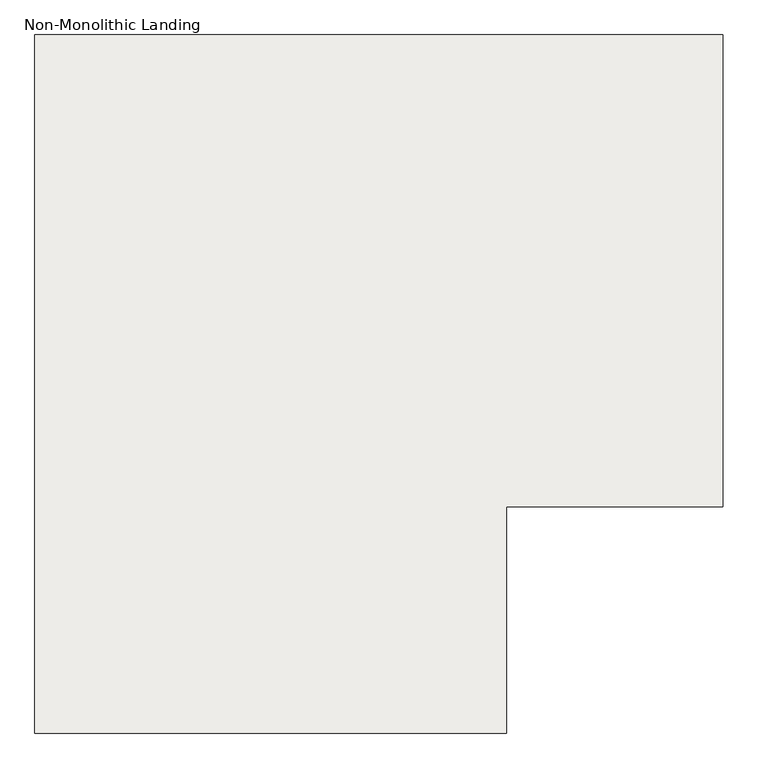
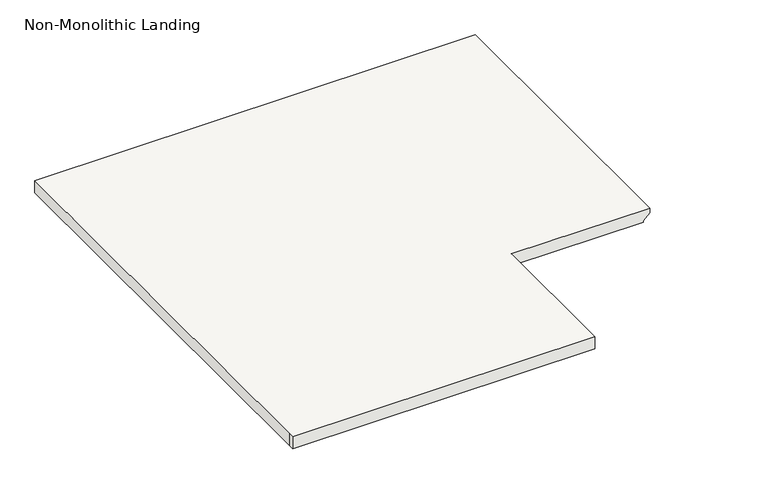
"""IFC4 building model written with IfcOpenShell, lengths in millimetres: slab geometry, Non-Monolithic Landing."""

import ifcopenshell
import ifcopenshell.guid

model = None  # the IFC model being written
_history = None  # IfcOwnerHistory: only IFC2X3 demands one
_inside = {}  # id of a spatial element -> (the spatial element, [elements in it])
_under = {}  # id of a project, library or spatial element -> (it, [spatial elements below it])
_declared = {}  # id of a project -> (the project, [libraries it declares])
_typed = {}  # id of a type object -> (the type object, [elements of that type])
_made_of = {}  # id of a material, layer set ... -> (it, [elements and type objects made of it])


def new_model(schema):
    """Start an empty IFC model of exactly this schema.

    Asked for "IFC4X3", IfcOpenShell would pick the latest addendum, in which some entities
    have other attributes; the version numbers below select the first issue.
    IFC2X3 requires an IfcOwnerHistory on every rooted entity: one is made here for all.
    """
    global model, _history
    if schema == "IFC4X3":
        model = ifcopenshell.file(schema_version=(4, 3, 0, 0))
    else:
        model = ifcopenshell.file(schema=schema)
    _inside.clear()
    _under.clear()
    _declared.clear()
    _typed.clear()
    _made_of.clear()
    _history = None
    if model.schema == "IFC2X3":
        org = make("IfcOrganization", Name="unknown")
        user = make(
            "IfcPersonAndOrganization",
            ThePerson=make("IfcPerson", FamilyName="unknown"),
            TheOrganization=org,
        )
        app = make(
            "IfcApplication",
            ApplicationDeveloper=org,
            Version="unknown",
            ApplicationFullName="unknown",
            ApplicationIdentifier="unknown",
        )
        _history = make(
            "IfcOwnerHistory",
            OwningUser=user,
            OwningApplication=app,
            ChangeAction="ADDED",
            CreationDate=0,
        )
    return model


def make(cls, **values):
    """One entity of the class cls with the attributes given. An attribute that is None is left unset."""
    return model.create_entity(
        cls, **{name: value for name, value in values.items() if value is not None}
    )


def rooted(cls, **values):
    """An entity with a GlobalId (a new one), such as an element, a storey or a relation."""
    return make(cls, GlobalId=ifcopenshell.guid.new(), OwnerHistory=_history, **values)


def si_unit(unit_type, name, prefix=None):
    """IfcSIUnit, for example si_unit("LENGTHUNIT", "METRE", prefix="MILLI")."""
    return make("IfcSIUnit", UnitType=unit_type, Prefix=prefix, Name=name)


def assignment(units):
    """IfcUnitAssignment: the units of a project."""
    return None if units is None else make("IfcUnitAssignment", Units=units)


def point(xyz):
    """IfcCartesianPoint."""
    return None if xyz is None else make("IfcCartesianPoint", Coordinates=xyz)


def direction(xyz):
    """IfcDirection."""
    return None if xyz is None else make("IfcDirection", DirectionRatios=xyz)


def frame(location, z_axis=None, x_axis=None):
    """IfcAxis2Placement3D, a coordinate frame: its origin and axes. An axis left out is left unset."""
    return make(
        "IfcAxis2Placement3D",
        Location=point(location),
        Axis=direction(z_axis),
        RefDirection=direction(x_axis),
    )


def origin():
    """The frame at (0, 0, 0) with its axes left unset."""
    return frame((0.0, 0.0, 0.0))


def place(relative_to, where):
    """IfcLocalPlacement: puts the frame where relative to a parent placement (None: the world)."""
    return make(
        "IfcLocalPlacement", PlacementRelTo=relative_to, RelativePlacement=where
    )


def context(
    kind, dimensions, precision=None, world=None, true_north=None, identifier=None
):
    """IfcGeometricRepresentationContext, for example the 3D "Model" context."""
    return make(
        "IfcGeometricRepresentationContext",
        ContextIdentifier=identifier,
        ContextType=kind,
        CoordinateSpaceDimension=dimensions,
        Precision=precision,
        WorldCoordinateSystem=world,
        TrueNorth=true_north,
    )


def project(units=None, contexts=None):
    """IfcProject with its units and contexts."""
    return rooted(
        "IfcProject",
        Name="project",
        RepresentationContexts=contexts,
        UnitsInContext=assignment(units),
    )


def spatial(cls, under=None, at=None, **own):
    """A site, building, storey or space (cls), placed at a placement, below another one or the project."""
    s = rooted(cls, ObjectPlacement=at, **own)
    if under is not None:
        _under.setdefault(under.id(), (under, []))[1].append(s)
    return s


def faces_of(points, faces, orient=None, outer=None):
    """IfcFace entities. A face is a list of loops; a loop is a list of indices into points, from 0.

    orient and outer hold one flag for each loop. By default every Orientation is true, the
    first loop of a face is its IfcFaceOuterBound and the others are IfcFaceBound.
    """
    made = []
    for i, loops in enumerate(faces):
        bounds = []
        for j, loop in enumerate(loops):
            is_outer = j == 0 if outer is None else outer[i][j]
            bounds.append(
                make(
                    "IfcFaceOuterBound" if is_outer else "IfcFaceBound",
                    Bound=make("IfcPolyLoop", Polygon=[points[k] for k in loop]),
                    Orientation=True if orient is None else orient[i][j],
                )
            )
        made.append(make("IfcFace", Bounds=bounds))
    return made


def faceted_brep(points, faces, orient=None, outer=None, voids=None):
    """IfcFacetedBrep: a solid bounded by flat faces; with voids (closed shells), ...WithVoids."""
    shared = [point(p) for p in points]
    hull = make("IfcClosedShell", CfsFaces=faces_of(shared, faces, orient, outer))
    if voids is None:
        return make("IfcFacetedBrep", Outer=hull)
    return make(
        "IfcFacetedBrepWithVoids",
        Outer=hull,
        Voids=[
            make(cls, CfsFaces=faces_of(shared, fs, o, b)) for cls, fs, o, b in voids
        ],
    )


def shape(context_of_items, identifier, shape_type, items):
    """IfcShapeRepresentation: the items that make up one representation, for example the "Body"."""
    return make(
        "IfcShapeRepresentation",
        ContextOfItems=context_of_items,
        RepresentationIdentifier=identifier,
        RepresentationType=shape_type,
        Items=items,
    )


def source(mapping_origin, context_of_items, identifier, shape_type, items):
    """IfcRepresentationMap: a shape defined once, which mapped items show again and again."""
    return make(
        "IfcRepresentationMap",
        MappingOrigin=mapping_origin,
        MappedRepresentation=shape(context_of_items, identifier, shape_type, items),
    )


def transform(
    local_origin,
    x_axis=None,
    y_axis=None,
    z_axis=None,
    scale=None,
    scale2=None,
    scale3=None,
    uniform=True,
):
    """IfcCartesianTransformationOperator3D, or its non-uniform kind. x_axis, y_axis, z_axis: its Axis1, 2, 3."""
    if uniform:
        return make(
            "IfcCartesianTransformationOperator3D",
            Axis1=direction(x_axis),
            Axis2=direction(y_axis),
            LocalOrigin=point(local_origin),
            Scale=scale,
            Axis3=direction(z_axis),
        )
    return make(
        "IfcCartesianTransformationOperator3DnonUniform",
        Axis1=direction(x_axis),
        Axis2=direction(y_axis),
        LocalOrigin=point(local_origin),
        Scale=scale,
        Axis3=direction(z_axis),
        Scale2=scale2,
        Scale3=scale3,
    )


def mapped(mapping_source, mapping_target):
    """IfcMappedItem: shows the shape of a source again, moved by a transform."""
    return make(
        "IfcMappedItem", MappingSource=mapping_source, MappingTarget=mapping_target
    )


def made_of(thing, what):
    """Note that an element or type object is made of a material, layer set ...; save() writes the relation."""
    if what is not None:
        _made_of.setdefault(what.id(), (what, []))[1].append(thing)
    return thing


def element(
    cls,
    number,
    at=None,
    inside=None,
    cuts=None,
    type_object=None,
    material=None,
    context=None,
    identifier="Body",
    shape_type=None,
    held_by="IfcProductDefinitionShape",
    body=None,
    shapes=None,
    **own,
):
    """One element of the class cls, such as IfcWall. Its Tag is "e" and its number.

    at: its placement. inside: the storey or other place that contains it. cuts: it is an
    opening in that element (IfcRelVoidsElement). A single representation is given by context,
    identifier, shape_type and body (its items); several are given by shapes. held_by: the class
    of the entity that holds the representations. save() writes the other relations.
    """
    e = rooted(cls, Tag="e%d" % number, ObjectPlacement=at, **own)
    if body is not None:
        shapes = [shape(context, identifier, shape_type, body)]
    if shapes is not None:
        e.Representation = make(held_by, Representations=shapes)
    if inside is not None:
        _inside.setdefault(inside.id(), (inside, []))[1].append(e)
    if cuts is not None:
        rooted(
            "IfcRelVoidsElement", RelatingBuildingElement=cuts, RelatedOpeningElement=e
        )
    if type_object is not None:
        _typed.setdefault(type_object.id(), (type_object, []))[1].append(e)
    return made_of(e, material)


def aggregate(whole, parts):
    """IfcRelAggregates: a whole, such as a stair, and the parts it consists of."""
    return rooted("IfcRelAggregates", RelatingObject=whole, RelatedObjects=parts)


def save(model, path):
    """Write the relations noted so far, then the file.

    IfcRelAggregates (storeys below a building ...), IfcRelContainedInSpatialStructure (elements
    in a storey), IfcRelDefinesByType, IfcRelAssociatesMaterial and IfcRelDeclares: one each for
    every whole, place, type object, material and project.
    """
    for whole, parts in _under.values():
        aggregate(whole, parts)
    for where, things in _inside.values():
        rooted(
            "IfcRelContainedInSpatialStructure",
            RelatedElements=things,
            RelatingStructure=where,
        )
    for kind, things in _typed.values():
        rooted("IfcRelDefinesByType", RelatedObjects=things, RelatingType=kind)
    for what, things in _made_of.values():
        rooted("IfcRelAssociatesMaterial", RelatedObjects=things, RelatingMaterial=what)
    for by, libraries in _declared.values():
        rooted("IfcRelDeclares", RelatingContext=by, RelatedDefinitions=libraries)
    model.write(path)


def non_monolithic_landing_74864503(model_context):
    return source(origin(), model_context, "Body", "Brep", [
        faceted_brep([(4668.4601743, -3020.5507921, 1200.15), (4668.4601743, -3020.5507921, 1219.2), (4668.4601743, -4239.7507921, 1219.2), (4668.4601743, -4239.7507921, 1200.15), (4643.0601743, -3020.5507921, 1174.75), (4643.0601743, -4239.7507921, 1174.75), (2890.4601743, -3020.5507921, 1219.2), (2890.4601743, -4798.5507921, 1219.2), (2890.4601743, -4823.9507921, 1219.2), (4109.6601743, -4823.9507921, 1219.2), (4109.6601743, -4798.5507921, 1219.2), (4109.6601743, -4239.7507921, 1219.2), (4643.0601743, -3020.5507921, 1168.4), (4643.0601743, -4239.7507921, 1168.4), (4109.6601743, -4239.7507921, 1168.4), (4109.6601743, -4798.5507921, 1168.4), (4109.6601743, -4823.9507921, 1168.4), (2890.4601743, -4823.9507921, 1168.4), (2890.4601743, -4798.5507921, 1168.4), (2890.4601743, -3020.5507921, 1168.4)], [[[0, 1, 2, 3]], [[4, 0, 3, 5]], [[6, 7, 8, 9, 10, 11, 2, 1]], [[12, 13, 14, 15, 16, 17, 18, 19]], [[13, 12, 4, 5]], [[6, 1, 0, 4, 12, 19]], [[7, 6, 19, 18]], [[8, 7, 18, 17]], [[9, 8, 17, 16]], [[10, 9, 16, 15]], [[11, 10, 15, 14]], [[2, 11, 14, 13, 5, 3]]]),
    ])


if __name__ == "__main__":
    model = new_model("IFC4")
    model_context = context("Model", 3, world=origin())
    ifc_project = project(units=[si_unit("LENGTHUNIT", "METRE", prefix="MILLI")], contexts=[model_context])
    site = spatial("IfcSite", under=ifc_project)
    building = spatial("IfcBuilding", under=site)
    placement = place(None, origin())
    non_monolithic_landing_shape = non_monolithic_landing_74864503(model_context)
    element("IfcSlab", 1, ObjectType="Non-Monolithic Landing", at=placement, inside=building, context=model_context, shape_type="MappedRepresentation", body=[
        mapped(non_monolithic_landing_shape, transform((0.0, 0.0, 0.0), x_axis=(1.0, 0.0, 0.0), y_axis=(0.0, 1.0, 0.0), z_axis=(0.0, 0.0, 1.0))),
    ])
    save(model, "model.ifc")

# Revit data of these elements
# Project information
#   Project Issue Date = "Issue Date"
#   Project Status = "Project Status"
#   Client Name = "Owner"
#   Project Address = "Enter address here"
#   Project Name = "Project Name"
#   Project Number = "Project Number"
